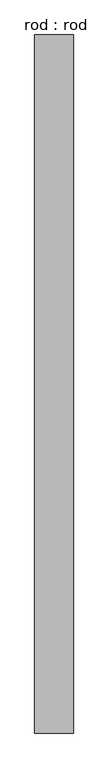
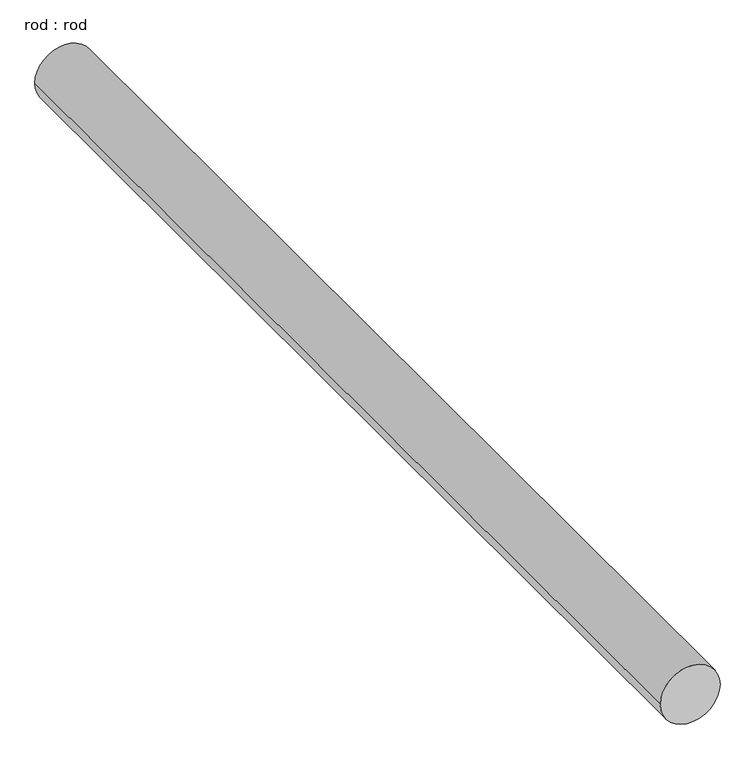
"""IFC4 building model written with IfcOpenShell, lengths in millimetres: proxy geometry, rod : rod."""

import ifcopenshell
import ifcopenshell.guid

model = None  # the IFC model being written
_history = None  # IfcOwnerHistory: only IFC2X3 demands one
_inside = {}  # id of a spatial element -> (the spatial element, [elements in it])
_under = {}  # id of a project, library or spatial element -> (it, [spatial elements below it])
_declared = {}  # id of a project -> (the project, [libraries it declares])
_typed = {}  # id of a type object -> (the type object, [elements of that type])
_made_of = {}  # id of a material, layer set ... -> (it, [elements and type objects made of it])


def new_model(schema):
    """Start an empty IFC model of exactly this schema.

    Asked for "IFC4X3", IfcOpenShell would pick the latest addendum, in which some entities
    have other attributes; the version numbers below select the first issue.
    IFC2X3 requires an IfcOwnerHistory on every rooted entity: one is made here for all.
    """
    global model, _history
    if schema == "IFC4X3":
        model = ifcopenshell.file(schema_version=(4, 3, 0, 0))
    else:
        model = ifcopenshell.file(schema=schema)
    _inside.clear()
    _under.clear()
    _declared.clear()
    _typed.clear()
    _made_of.clear()
    _history = None
    if model.schema == "IFC2X3":
        org = make("IfcOrganization", Name="unknown")
        user = make(
            "IfcPersonAndOrganization",
            ThePerson=make("IfcPerson", FamilyName="unknown"),
            TheOrganization=org,
        )
        app = make(
            "IfcApplication",
            ApplicationDeveloper=org,
            Version="unknown",
            ApplicationFullName="unknown",
            ApplicationIdentifier="unknown",
        )
        _history = make(
            "IfcOwnerHistory",
            OwningUser=user,
            OwningApplication=app,
            ChangeAction="ADDED",
            CreationDate=0,
        )
    return model


def make(cls, **values):
    """One entity of the class cls with the attributes given. An attribute that is None is left unset."""
    return model.create_entity(
        cls, **{name: value for name, value in values.items() if value is not None}
    )


def rooted(cls, **values):
    """An entity with a GlobalId (a new one), such as an element, a storey or a relation."""
    return make(cls, GlobalId=ifcopenshell.guid.new(), OwnerHistory=_history, **values)


def si_unit(unit_type, name, prefix=None):
    """IfcSIUnit, for example si_unit("LENGTHUNIT", "METRE", prefix="MILLI")."""
    return make("IfcSIUnit", UnitType=unit_type, Prefix=prefix, Name=name)


def assignment(units):
    """IfcUnitAssignment: the units of a project."""
    return None if units is None else make("IfcUnitAssignment", Units=units)


def point(xyz):
    """IfcCartesianPoint."""
    return None if xyz is None else make("IfcCartesianPoint", Coordinates=xyz)


def direction(xyz):
    """IfcDirection."""
    return None if xyz is None else make("IfcDirection", DirectionRatios=xyz)


def frame(location, z_axis=None, x_axis=None):
    """IfcAxis2Placement3D, a coordinate frame: its origin and axes. An axis left out is left unset."""
    return make(
        "IfcAxis2Placement3D",
        Location=point(location),
        Axis=direction(z_axis),
        RefDirection=direction(x_axis),
    )


def frame_2d(location, x_axis=None):
    """IfcAxis2Placement2D, a coordinate frame in the plane: its origin and x axis."""
    return make(
        "IfcAxis2Placement2D", Location=point(location), RefDirection=direction(x_axis)
    )


def origin():
    """The frame at (0, 0, 0) with its axes left unset."""
    return frame((0.0, 0.0, 0.0))


def place(relative_to, where):
    """IfcLocalPlacement: puts the frame where relative to a parent placement (None: the world)."""
    return make(
        "IfcLocalPlacement", PlacementRelTo=relative_to, RelativePlacement=where
    )


def context(
    kind, dimensions, precision=None, world=None, true_north=None, identifier=None
):
    """IfcGeometricRepresentationContext, for example the 3D "Model" context."""
    return make(
        "IfcGeometricRepresentationContext",
        ContextIdentifier=identifier,
        ContextType=kind,
        CoordinateSpaceDimension=dimensions,
        Precision=precision,
        WorldCoordinateSystem=world,
        TrueNorth=true_north,
    )


def project(units=None, contexts=None):
    """IfcProject with its units and contexts."""
    return rooted(
        "IfcProject",
        Name="project",
        RepresentationContexts=contexts,
        UnitsInContext=assignment(units),
    )


def spatial(cls, under=None, at=None, **own):
    """A site, building, storey or space (cls), placed at a placement, below another one or the project."""
    s = rooted(cls, ObjectPlacement=at, **own)
    if under is not None:
        _under.setdefault(under.id(), (under, []))[1].append(s)
    return s


def circle_curve(where, radius):
    """IfcCircle in the frame where."""
    return make("IfcCircle", Position=where, Radius=radius)


def trimmed(basis, trim1, trim2, sense, master):
    """IfcTrimmedCurve: the piece of a basis curve between two trims."""
    return make(
        "IfcTrimmedCurve",
        BasisCurve=basis,
        Trim1=trim1,
        Trim2=trim2,
        SenseAgreement=sense,
        MasterRepresentation=master,
    )


def segment(curve, same_sense, transition):
    """IfcCompositeCurveSegment."""
    return make(
        "IfcCompositeCurveSegment",
        Transition=transition,
        SameSense=same_sense,
        ParentCurve=curve,
    )


def composite_curve(segments, self_intersect=None):
    """IfcCompositeCurve: segments joined end to end."""
    return make("IfcCompositeCurve", Segments=segments, SelfIntersect=self_intersect)


def outline(outer, holes=None, kind="AREA"):
    """IfcArbitraryClosedProfileDef: a profile drawn as a closed curve; with holes, ...WithVoids."""
    if holes is None:
        return make("IfcArbitraryClosedProfileDef", ProfileType=kind, OuterCurve=outer)
    return make(
        "IfcArbitraryProfileDefWithVoids",
        ProfileType=kind,
        OuterCurve=outer,
        InnerCurves=holes,
    )


def extrude(swept, where, along, depth):
    """IfcExtrudedAreaSolid: the profile swept, set in the frame where, extruded along a direction by depth."""
    return make(
        "IfcExtrudedAreaSolid",
        SweptArea=swept,
        Position=where,
        ExtrudedDirection=direction(along),
        Depth=depth,
    )


def shape(context_of_items, identifier, shape_type, items):
    """IfcShapeRepresentation: the items that make up one representation, for example the "Body"."""
    return make(
        "IfcShapeRepresentation",
        ContextOfItems=context_of_items,
        RepresentationIdentifier=identifier,
        RepresentationType=shape_type,
        Items=items,
    )


def source(mapping_origin, context_of_items, identifier, shape_type, items):
    """IfcRepresentationMap: a shape defined once, which mapped items show again and again."""
    return make(
        "IfcRepresentationMap",
        MappingOrigin=mapping_origin,
        MappedRepresentation=shape(context_of_items, identifier, shape_type, items),
    )


def transform(
    local_origin,
    x_axis=None,
    y_axis=None,
    z_axis=None,
    scale=None,
    scale2=None,
    scale3=None,
    uniform=True,
):
    """IfcCartesianTransformationOperator3D, or its non-uniform kind. x_axis, y_axis, z_axis: its Axis1, 2, 3."""
    if uniform:
        return make(
            "IfcCartesianTransformationOperator3D",
            Axis1=direction(x_axis),
            Axis2=direction(y_axis),
            LocalOrigin=point(local_origin),
            Scale=scale,
            Axis3=direction(z_axis),
        )
    return make(
        "IfcCartesianTransformationOperator3DnonUniform",
        Axis1=direction(x_axis),
        Axis2=direction(y_axis),
        LocalOrigin=point(local_origin),
        Scale=scale,
        Axis3=direction(z_axis),
        Scale2=scale2,
        Scale3=scale3,
    )


def mapped(mapping_source, mapping_target):
    """IfcMappedItem: shows the shape of a source again, moved by a transform."""
    return make(
        "IfcMappedItem", MappingSource=mapping_source, MappingTarget=mapping_target
    )


def made_of(thing, what):
    """Note that an element or type object is made of a material, layer set ...; save() writes the relation."""
    if what is not None:
        _made_of.setdefault(what.id(), (what, []))[1].append(thing)
    return thing


def element(
    cls,
    number,
    at=None,
    inside=None,
    cuts=None,
    type_object=None,
    material=None,
    context=None,
    identifier="Body",
    shape_type=None,
    held_by="IfcProductDefinitionShape",
    body=None,
    shapes=None,
    **own,
):
    """One element of the class cls, such as IfcWall. Its Tag is "e" and its number.

    at: its placement. inside: the storey or other place that contains it. cuts: it is an
    opening in that element (IfcRelVoidsElement). A single representation is given by context,
    identifier, shape_type and body (its items); several are given by shapes. held_by: the class
    of the entity that holds the representations. save() writes the other relations.
    """
    e = rooted(cls, Tag="e%d" % number, ObjectPlacement=at, **own)
    if body is not None:
        shapes = [shape(context, identifier, shape_type, body)]
    if shapes is not None:
        e.Representation = make(held_by, Representations=shapes)
    if inside is not None:
        _inside.setdefault(inside.id(), (inside, []))[1].append(e)
    if cuts is not None:
        rooted(
            "IfcRelVoidsElement", RelatingBuildingElement=cuts, RelatedOpeningElement=e
        )
    if type_object is not None:
        _typed.setdefault(type_object.id(), (type_object, []))[1].append(e)
    return made_of(e, material)


def aggregate(whole, parts):
    """IfcRelAggregates: a whole, such as a stair, and the parts it consists of."""
    return rooted("IfcRelAggregates", RelatingObject=whole, RelatedObjects=parts)


def save(model, path):
    """Write the relations noted so far, then the file.

    IfcRelAggregates (storeys below a building ...), IfcRelContainedInSpatialStructure (elements
    in a storey), IfcRelDefinesByType, IfcRelAssociatesMaterial and IfcRelDeclares: one each for
    every whole, place, type object, material and project.
    """
    for whole, parts in _under.values():
        aggregate(whole, parts)
    for where, things in _inside.values():
        rooted(
            "IfcRelContainedInSpatialStructure",
            RelatedElements=things,
            RelatingStructure=where,
        )
    for kind, things in _typed.values():
        rooted("IfcRelDefinesByType", RelatedObjects=things, RelatingType=kind)
    for what, things in _made_of.values():
        rooted("IfcRelAssociatesMaterial", RelatedObjects=things, RelatingMaterial=what)
    for by, libraries in _declared.values():
        rooted("IfcRelDeclares", RelatingContext=by, RelatedDefinitions=libraries)
    model.write(path)


def rod_rod_d274bac8(model_context):
    return source(origin(), model_context, "Body", "SweptSolid", [
        extrude(outline(composite_curve([segment(trimmed(circle_curve(frame_2d((0.0108462, 0.0)), 200.0), [point((0.0108462, 200.0))], [point((0.0108462, -200.0))], False, "CARTESIAN"), True, "CONTINUOUS"), segment(trimmed(circle_curve(frame_2d((0.0108462, 0.0)), 200.0), [point((0.0108462, -200.0))], [point((0.0108462, 200.0))], False, "CARTESIAN"), True, "CONTINUOUS")], self_intersect=False)), frame((0.0, 477.617967, 0.0), z_axis=(0.0, 1.0, 0.0), x_axis=(0.0, 0.0, 1.0)), (0.0, 0.0, 1.0), 7230.2212968),
    ])


if __name__ == "__main__":
    model = new_model("IFC4")
    model_context = context("Model", 3, world=origin())
    ifc_project = project(units=[si_unit("LENGTHUNIT", "METRE", prefix="MILLI")], contexts=[model_context])
    site = spatial("IfcSite", under=ifc_project)
    building = spatial("IfcBuilding", under=site)
    placement = place(None, origin())
    rod_rod_shape = rod_rod_d274bac8(model_context)
    element("IfcBuildingElementProxy", 1, Name="rod : rod", ObjectType="rod : rod", at=placement, inside=building, context=model_context, shape_type="MappedRepresentation", body=[
        mapped(rod_rod_shape, transform((0.0, 0.0, 0.0), x_axis=(1.0, 0.0, 0.0), y_axis=(0.0, 1.0, 0.0), z_axis=(0.0, 0.0, 1.0))),
    ])
    save(model, "model.ifc")

# Revit data of these elements
# Type "rod : rod"
#   Default Elevation = 0
